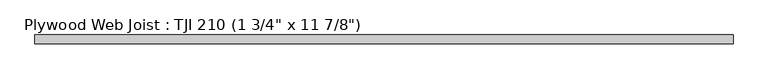
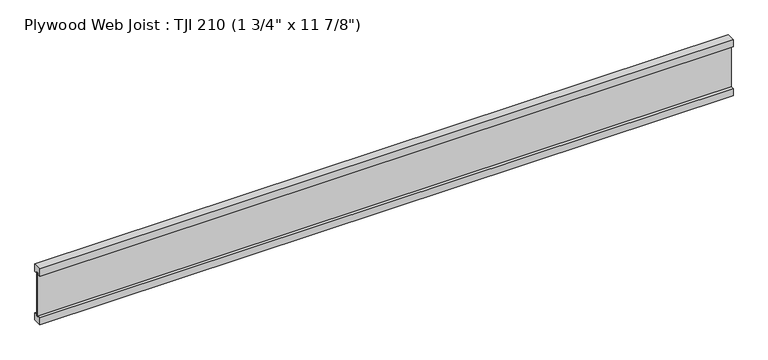
"""IFC4 building model written with IfcOpenShell, lengths in millimetres: beam geometry."""

from ifc_helpers import new_model, si_unit, frame, origin, place, context, project, spatial, polyline, outline, extrude, source, transform, mapped, element, save


def beam_ee03622c(model_context):
    return source(origin(), model_context, "Body", "SweptSolid", [
        extrude(outline(polyline([(-22.225, 150.8125), (22.225, 150.8125), (22.225, 112.7125), (4.7625, 112.7125), (4.7625, 119.0625), (-4.7625, 119.0625), (-4.7625, 112.7125), (-22.225, 112.7125), (-22.225, 150.8125)])), frame((-1787.525, 0.0, 0.0), z_axis=(1.0, 0.0, 0.0), x_axis=(0.0, 1.0, 0.0)), (0.0, 0.0, 1.0), 3530.6),
        extrude(outline(polyline([(22.225, -112.7125), (22.225, -150.8125), (-22.225, -150.8125), (-22.225, -112.7125), (-4.7625, -112.7125), (-4.7625, -118.3285374), (4.7625, -118.3285374), (4.7625, -112.7125), (22.225, -112.7125)])), frame((-1787.525, 0.0, 0.0), z_axis=(1.0, 0.0, 0.0), x_axis=(0.0, 1.0, 0.0)), (0.0, 0.0, 1.0), 3530.6),
        extrude(outline(polyline([(1743.075, 4.7625), (1743.075, -4.7625), (-1787.525, -4.7625), (-1787.525, 4.7625), (1743.075, 4.7625)])), frame((0.0, 0.0, -118.3285374), z_axis=(0.0, 0.0, 1.0), x_axis=(1.0, 0.0, 0.0)), (0.0, 0.0, 1.0), 237.3910374),
    ])


if __name__ == "__main__":
    model = new_model("IFC4")
    model_context = context("Model", 3, world=origin())
    ifc_project = project(units=[si_unit("LENGTHUNIT", "METRE", prefix="MILLI")], contexts=[model_context])
    site = spatial("IfcSite", under=ifc_project)
    building = spatial("IfcBuilding", under=site)
    placement = place(None, origin())
    beam_shape = beam_ee03622c(model_context)
    element("IfcBeam", 1, ObjectType="Plywood Web Joist : TJI 210 (1 3/4\" x 11 7/8\")", at=placement, inside=building, context=model_context, shape_type="MappedRepresentation", body=[
        mapped(beam_shape, transform((0.0, 0.0, 0.0), x_axis=(1.0, 0.0, 0.0), y_axis=(0.0, 1.0, 0.0), z_axis=(0.0, 0.0, 1.0))),
    ])
    save(model, "model.ifc")

# Revit data of these elements
# Type "Plywood Web Joist : TJI 210 (1 3/4\" x 11 7/8\")"
#   Assembly Code = "B10"
#   Length [instance default] = 5' - 0"
#   b = 0' - 1 3/4"
#   d = 0' - 11 7/8"
#   Structural Material [instance default] = Softwood, Lumber
# Element 1 (IfcBeam, "Plywood Web Joist : TJI 210 (1 3/4\" x 11 7/8\")")
#   Materials on its faces: "Softwood, Lumber"
# Materials
#   "Softwood, Lumber": class "Wood", colour RGB 144 113 62, transparency 0, Description = "Pinus Echinata", Cost = 0
